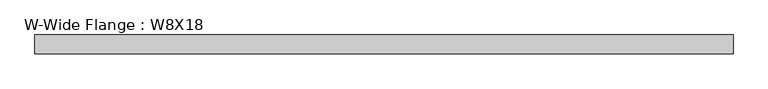
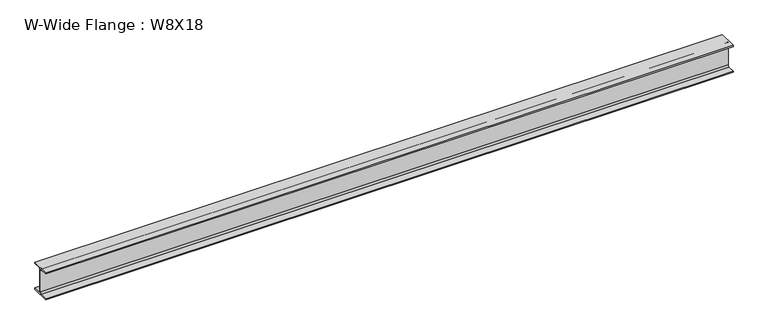
"""IFC4 building model written with IfcOpenShell, lengths in millimetres: beam geometry, W-Wide Flange : W8X18."""

from ifc_helpers import new_model, si_unit, point, frame, frame_2d, origin, place, context, project, spatial, polyline, circle_curve, trimmed, segment, composite_curve, outline, extrude, source, transform, mapped, element, save


def w_wide_flange_w8x18_62c2d6be(model_context):
    return source(origin(), model_context, "Body", "SweptSolid", [
        extrude(outline(composite_curve([segment(polyline([(66.675, -94.996), (66.675, -103.378), (-66.675, -103.378), (-66.675, -94.996), (-15.1765, -94.996)]), True, "CONTINUOUS"), segment(trimmed(circle_curve(frame_2d((-15.1765, -82.7405)), 12.2555), [point((-15.1765, -94.996))], [point((-2.921, -82.7405))], True, "CARTESIAN"), True, "CONTINUOUS"), segment(polyline([(-2.921, -82.7405), (-2.921, 82.7405)]), True, "CONTINUOUS"), segment(trimmed(circle_curve(frame_2d((-15.1765, 82.7405)), 12.2555), [point((-2.921, 82.7405))], [point((-15.1765, 94.996))], True, "CARTESIAN"), True, "CONTINUOUS"), segment(polyline([(-15.1765, 94.996), (-66.675, 94.996), (-66.675, 103.378), (66.675, 103.378), (66.675, 94.996), (15.1765, 94.996)]), True, "CONTINUOUS"), segment(trimmed(circle_curve(frame_2d((15.1765, 82.7405)), 12.2555), [point((15.1765, 94.996))], [point((2.921, 82.7405))], True, "CARTESIAN"), True, "CONTINUOUS"), segment(polyline([(2.921, 82.7405), (2.921, -82.7405)]), True, "CONTINUOUS"), segment(trimmed(circle_curve(frame_2d((15.1765, -82.7405)), 12.2555), [point((2.921, -82.7405))], [point((15.1765, -94.996))], True, "CARTESIAN"), True, "CONTINUOUS"), segment(polyline([(15.1765, -94.996), (66.675, -94.996)]), True, "CONTINUOUS")], self_intersect=False)), frame((-2467.4266146, 0.0, 0.0), z_axis=(1.0, 0.0, 0.0), x_axis=(0.0, 1.0, 0.0)), (0.0, 0.0, 1.0), 4982.2695313),
    ])


if __name__ == "__main__":
    model = new_model("IFC4")
    model_context = context("Model", 3, world=origin())
    ifc_project = project(units=[si_unit("LENGTHUNIT", "METRE", prefix="MILLI")], contexts=[model_context])
    site = spatial("IfcSite", under=ifc_project)
    building = spatial("IfcBuilding", under=site)
    placement = place(None, origin())
    w_wide_flange_w8x18_shape = w_wide_flange_w8x18_62c2d6be(model_context)
    element("IfcBeam", 1, ObjectType="W-Wide Flange : W8X18", at=placement, inside=building, context=model_context, shape_type="MappedRepresentation", body=[
        mapped(w_wide_flange_w8x18_shape, transform((0.0, 0.0, 0.0), x_axis=(1.0, 0.0, 0.0), y_axis=(0.0, 1.0, 0.0), z_axis=(0.0, 0.0, 1.0))),
    ])
    save(model, "model.ifc")

# Revit data of these elements
# Type "W-Wide Flange : W8X18"
#   Assembly Code = "B10"
#   W = 18
#   Length [instance default] = 1524 mm
#   bf = 133.35 mm
#   d = 206.756 mm
#   k = 20.638 mm
#   k2 = 12.256 mm
#   tf = 8.382 mm
#   tw = 5.842 mm
#   A = 0.00339354 m²
#   Structural Material [instance default] = Steel ASTM A992
# Element 1 (IfcBeam, "W-Wide Flange : W8X18")
#   Structural Material = Aluminum, Anodized Red
#   Materials on its faces: "Aluminum, Anodized Red"
# Materials
#   "Steel ASTM A992": class "Metal", colour RGB 128 0 0, transparency 0, Description = "Structural steel 50ksi", Cost = 0
#   "Aluminum, Anodized Red": class "Metal", colour RGB 120 120 120, transparency 0, Description = "Anodized aluminum, red", Cost = 0
